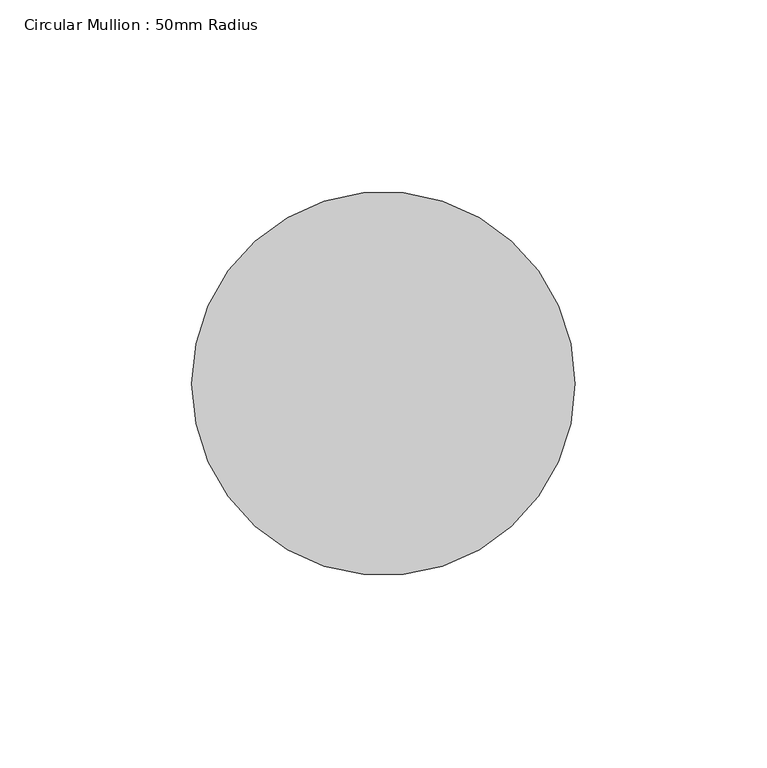
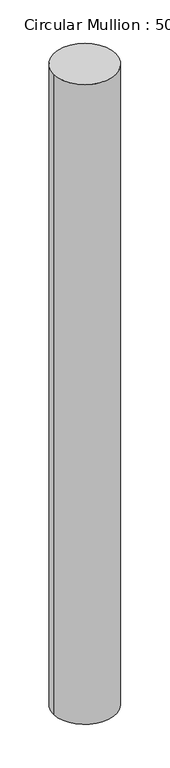
"""IFC4 building model written with IfcOpenShell, lengths in millimetres: member geometry, Circular Mullion : 50mm Radius."""

import ifcopenshell
import ifcopenshell.guid

model = None  # the IFC model being written
_history = None  # IfcOwnerHistory: only IFC2X3 demands one
_inside = {}  # id of a spatial element -> (the spatial element, [elements in it])
_under = {}  # id of a project, library or spatial element -> (it, [spatial elements below it])
_declared = {}  # id of a project -> (the project, [libraries it declares])
_typed = {}  # id of a type object -> (the type object, [elements of that type])
_made_of = {}  # id of a material, layer set ... -> (it, [elements and type objects made of it])


def new_model(schema):
    """Start an empty IFC model of exactly this schema.

    Asked for "IFC4X3", IfcOpenShell would pick the latest addendum, in which some entities
    have other attributes; the version numbers below select the first issue.
    IFC2X3 requires an IfcOwnerHistory on every rooted entity: one is made here for all.
    """
    global model, _history
    if schema == "IFC4X3":
        model = ifcopenshell.file(schema_version=(4, 3, 0, 0))
    else:
        model = ifcopenshell.file(schema=schema)
    _inside.clear()
    _under.clear()
    _declared.clear()
    _typed.clear()
    _made_of.clear()
    _history = None
    if model.schema == "IFC2X3":
        org = make("IfcOrganization", Name="unknown")
        user = make(
            "IfcPersonAndOrganization",
            ThePerson=make("IfcPerson", FamilyName="unknown"),
            TheOrganization=org,
        )
        app = make(
            "IfcApplication",
            ApplicationDeveloper=org,
            Version="unknown",
            ApplicationFullName="unknown",
            ApplicationIdentifier="unknown",
        )
        _history = make(
            "IfcOwnerHistory",
            OwningUser=user,
            OwningApplication=app,
            ChangeAction="ADDED",
            CreationDate=0,
        )
    return model


def make(cls, **values):
    """One entity of the class cls with the attributes given. An attribute that is None is left unset."""
    return model.create_entity(
        cls, **{name: value for name, value in values.items() if value is not None}
    )


def rooted(cls, **values):
    """An entity with a GlobalId (a new one), such as an element, a storey or a relation."""
    return make(cls, GlobalId=ifcopenshell.guid.new(), OwnerHistory=_history, **values)


def si_unit(unit_type, name, prefix=None):
    """IfcSIUnit, for example si_unit("LENGTHUNIT", "METRE", prefix="MILLI")."""
    return make("IfcSIUnit", UnitType=unit_type, Prefix=prefix, Name=name)


def assignment(units):
    """IfcUnitAssignment: the units of a project."""
    return None if units is None else make("IfcUnitAssignment", Units=units)


def point(xyz):
    """IfcCartesianPoint."""
    return None if xyz is None else make("IfcCartesianPoint", Coordinates=xyz)


def direction(xyz):
    """IfcDirection."""
    return None if xyz is None else make("IfcDirection", DirectionRatios=xyz)


def frame(location, z_axis=None, x_axis=None):
    """IfcAxis2Placement3D, a coordinate frame: its origin and axes. An axis left out is left unset."""
    return make(
        "IfcAxis2Placement3D",
        Location=point(location),
        Axis=direction(z_axis),
        RefDirection=direction(x_axis),
    )


def frame_2d(location, x_axis=None):
    """IfcAxis2Placement2D, a coordinate frame in the plane: its origin and x axis."""
    return make(
        "IfcAxis2Placement2D", Location=point(location), RefDirection=direction(x_axis)
    )


def origin():
    """The frame at (0, 0, 0) with its axes left unset."""
    return frame((0.0, 0.0, 0.0))


def origin_2d():
    """The frame at (0, 0) in the plane with its x axis left unset."""
    return frame_2d((0.0, 0.0))


def place(relative_to, where):
    """IfcLocalPlacement: puts the frame where relative to a parent placement (None: the world)."""
    return make(
        "IfcLocalPlacement", PlacementRelTo=relative_to, RelativePlacement=where
    )


def context(
    kind, dimensions, precision=None, world=None, true_north=None, identifier=None
):
    """IfcGeometricRepresentationContext, for example the 3D "Model" context."""
    return make(
        "IfcGeometricRepresentationContext",
        ContextIdentifier=identifier,
        ContextType=kind,
        CoordinateSpaceDimension=dimensions,
        Precision=precision,
        WorldCoordinateSystem=world,
        TrueNorth=true_north,
    )


def project(units=None, contexts=None):
    """IfcProject with its units and contexts."""
    return rooted(
        "IfcProject",
        Name="project",
        RepresentationContexts=contexts,
        UnitsInContext=assignment(units),
    )


def spatial(cls, under=None, at=None, **own):
    """A site, building, storey or space (cls), placed at a placement, below another one or the project."""
    s = rooted(cls, ObjectPlacement=at, **own)
    if under is not None:
        _under.setdefault(under.id(), (under, []))[1].append(s)
    return s


def circle_curve(where, radius):
    """IfcCircle in the frame where."""
    return make("IfcCircle", Position=where, Radius=radius)


def trimmed(basis, trim1, trim2, sense, master):
    """IfcTrimmedCurve: the piece of a basis curve between two trims."""
    return make(
        "IfcTrimmedCurve",
        BasisCurve=basis,
        Trim1=trim1,
        Trim2=trim2,
        SenseAgreement=sense,
        MasterRepresentation=master,
    )


def segment(curve, same_sense, transition):
    """IfcCompositeCurveSegment."""
    return make(
        "IfcCompositeCurveSegment",
        Transition=transition,
        SameSense=same_sense,
        ParentCurve=curve,
    )


def composite_curve(segments, self_intersect=None):
    """IfcCompositeCurve: segments joined end to end."""
    return make("IfcCompositeCurve", Segments=segments, SelfIntersect=self_intersect)


def outline(outer, holes=None, kind="AREA"):
    """IfcArbitraryClosedProfileDef: a profile drawn as a closed curve; with holes, ...WithVoids."""
    if holes is None:
        return make("IfcArbitraryClosedProfileDef", ProfileType=kind, OuterCurve=outer)
    return make(
        "IfcArbitraryProfileDefWithVoids",
        ProfileType=kind,
        OuterCurve=outer,
        InnerCurves=holes,
    )


def extrude(swept, where, along, depth):
    """IfcExtrudedAreaSolid: the profile swept, set in the frame where, extruded along a direction by depth."""
    return make(
        "IfcExtrudedAreaSolid",
        SweptArea=swept,
        Position=where,
        ExtrudedDirection=direction(along),
        Depth=depth,
    )


def shape(context_of_items, identifier, shape_type, items):
    """IfcShapeRepresentation: the items that make up one representation, for example the "Body"."""
    return make(
        "IfcShapeRepresentation",
        ContextOfItems=context_of_items,
        RepresentationIdentifier=identifier,
        RepresentationType=shape_type,
        Items=items,
    )


def source(mapping_origin, context_of_items, identifier, shape_type, items):
    """IfcRepresentationMap: a shape defined once, which mapped items show again and again."""
    return make(
        "IfcRepresentationMap",
        MappingOrigin=mapping_origin,
        MappedRepresentation=shape(context_of_items, identifier, shape_type, items),
    )


def transform(
    local_origin,
    x_axis=None,
    y_axis=None,
    z_axis=None,
    scale=None,
    scale2=None,
    scale3=None,
    uniform=True,
):
    """IfcCartesianTransformationOperator3D, or its non-uniform kind. x_axis, y_axis, z_axis: its Axis1, 2, 3."""
    if uniform:
        return make(
            "IfcCartesianTransformationOperator3D",
            Axis1=direction(x_axis),
            Axis2=direction(y_axis),
            LocalOrigin=point(local_origin),
            Scale=scale,
            Axis3=direction(z_axis),
        )
    return make(
        "IfcCartesianTransformationOperator3DnonUniform",
        Axis1=direction(x_axis),
        Axis2=direction(y_axis),
        LocalOrigin=point(local_origin),
        Scale=scale,
        Axis3=direction(z_axis),
        Scale2=scale2,
        Scale3=scale3,
    )


def mapped(mapping_source, mapping_target):
    """IfcMappedItem: shows the shape of a source again, moved by a transform."""
    return make(
        "IfcMappedItem", MappingSource=mapping_source, MappingTarget=mapping_target
    )


def made_of(thing, what):
    """Note that an element or type object is made of a material, layer set ...; save() writes the relation."""
    if what is not None:
        _made_of.setdefault(what.id(), (what, []))[1].append(thing)
    return thing


def element(
    cls,
    number,
    at=None,
    inside=None,
    cuts=None,
    type_object=None,
    material=None,
    context=None,
    identifier="Body",
    shape_type=None,
    held_by="IfcProductDefinitionShape",
    body=None,
    shapes=None,
    **own,
):
    """One element of the class cls, such as IfcWall. Its Tag is "e" and its number.

    at: its placement. inside: the storey or other place that contains it. cuts: it is an
    opening in that element (IfcRelVoidsElement). A single representation is given by context,
    identifier, shape_type and body (its items); several are given by shapes. held_by: the class
    of the entity that holds the representations. save() writes the other relations.
    """
    e = rooted(cls, Tag="e%d" % number, ObjectPlacement=at, **own)
    if body is not None:
        shapes = [shape(context, identifier, shape_type, body)]
    if shapes is not None:
        e.Representation = make(held_by, Representations=shapes)
    if inside is not None:
        _inside.setdefault(inside.id(), (inside, []))[1].append(e)
    if cuts is not None:
        rooted(
            "IfcRelVoidsElement", RelatingBuildingElement=cuts, RelatedOpeningElement=e
        )
    if type_object is not None:
        _typed.setdefault(type_object.id(), (type_object, []))[1].append(e)
    return made_of(e, material)


def aggregate(whole, parts):
    """IfcRelAggregates: a whole, such as a stair, and the parts it consists of."""
    return rooted("IfcRelAggregates", RelatingObject=whole, RelatedObjects=parts)


def save(model, path):
    """Write the relations noted so far, then the file.

    IfcRelAggregates (storeys below a building ...), IfcRelContainedInSpatialStructure (elements
    in a storey), IfcRelDefinesByType, IfcRelAssociatesMaterial and IfcRelDeclares: one each for
    every whole, place, type object, material and project.
    """
    for whole, parts in _under.values():
        aggregate(whole, parts)
    for where, things in _inside.values():
        rooted(
            "IfcRelContainedInSpatialStructure",
            RelatedElements=things,
            RelatingStructure=where,
        )
    for kind, things in _typed.values():
        rooted("IfcRelDefinesByType", RelatedObjects=things, RelatingType=kind)
    for what, things in _made_of.values():
        rooted("IfcRelAssociatesMaterial", RelatedObjects=things, RelatingMaterial=what)
    for by, libraries in _declared.values():
        rooted("IfcRelDeclares", RelatingContext=by, RelatedDefinitions=libraries)
    model.write(path)


def circular_mullion_50mm_radius_b22df4d7(model_context):
    return source(origin(), model_context, "Body", "SweptSolid", [
        extrude(outline(composite_curve([segment(trimmed(circle_curve(origin_2d(), 50.0), [point((50.0, 0.0))], [point((-50.0, 0.0))], False, "CARTESIAN"), True, "CONTINUOUS"), segment(trimmed(circle_curve(origin_2d(), 50.0), [point((-50.0, 0.0))], [point((50.0, 0.0))], False, "CARTESIAN"), True, "CONTINUOUS")], self_intersect=False)), frame((0.0, 0.0, -1086.9414004), z_axis=(0.0, 0.0, 1.0), x_axis=(1.0, 0.0, 0.0)), (0.0, 0.0, 1.0), 1086.9414004),
    ])


if __name__ == "__main__":
    model = new_model("IFC4")
    model_context = context("Model", 3, world=origin())
    ifc_project = project(units=[si_unit("LENGTHUNIT", "METRE", prefix="MILLI")], contexts=[model_context])
    site = spatial("IfcSite", under=ifc_project)
    building = spatial("IfcBuilding", under=site)
    placement = place(None, origin())
    circular_mullion_50mm_radius_shape = circular_mullion_50mm_radius_b22df4d7(model_context)
    element("IfcMember", 1, ObjectType="Circular Mullion : 50mm Radius", at=placement, inside=building, context=model_context, shape_type="MappedRepresentation", body=[
        mapped(circular_mullion_50mm_radius_shape, transform((0.0, 0.0, 0.0), x_axis=(1.0, 0.0, 0.0), y_axis=(0.0, 1.0, 0.0), z_axis=(0.0, 0.0, 1.0))),
    ])
    save(model, "model.ifc")

# Revit data of these elements
# Type "Circular Mullion : 50mm Radius"
#   built-in parameter 1007350 = 0.164042 (stored number, unit not read)
# Element 1 (IfcMember, "Circular Mullion : 50mm Radius")
#   Materials on its faces: "Aluminium"
# Materials
#   "Aluminium": class "Metal", colour RGB 247 247 247, transparency 0, Description = "Aluminium 6061", Cost = 0
